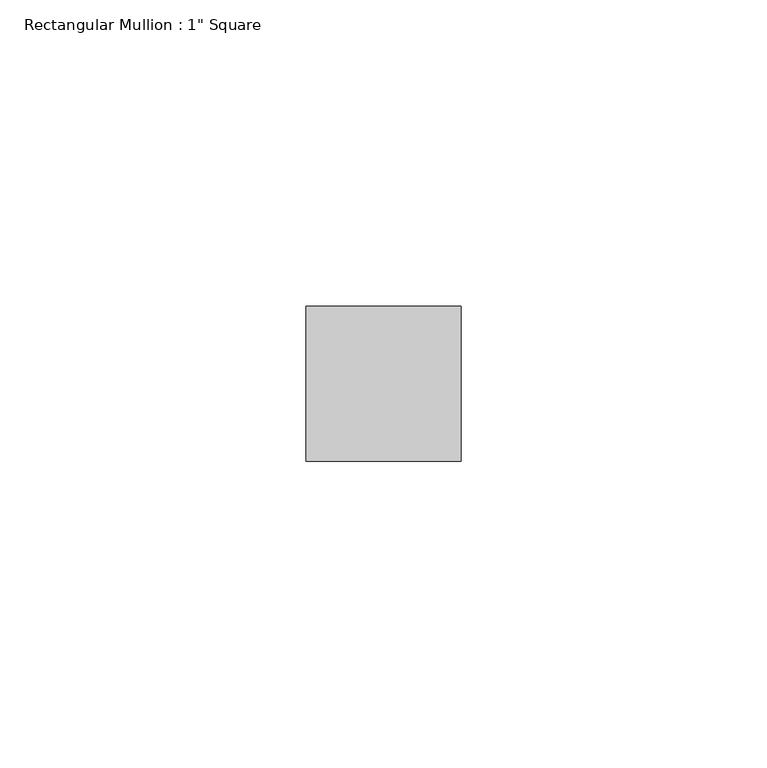
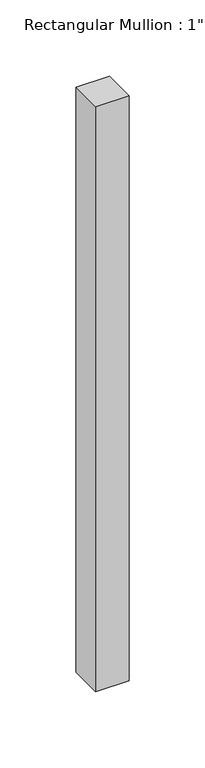
"""IFC4 building model written with IfcOpenShell, lengths in millimetres: member geometry."""

from ifc_helpers import new_model, si_unit, frame, origin, place, context, project, spatial, polyline, outline, extrude, source, transform, mapped, element, save


def member_0282b000(model_context):
    return source(origin(), model_context, "Body", "SweptSolid", [
        extrude(outline(polyline([(0.0, 12.7), (0.0, -12.7), (-25.4, -12.7), (-25.4, 12.7), (0.0, 12.7)])), frame((0.0, 0.0, -468.2712073), z_axis=(0.0, 0.0, 1.0), x_axis=(1.0, 0.0, 0.0)), (0.0, 0.0, 1.0), 468.2712073),
    ])


if __name__ == "__main__":
    model = new_model("IFC4")
    model_context = context("Model", 3, world=origin())
    ifc_project = project(units=[si_unit("LENGTHUNIT", "METRE", prefix="MILLI")], contexts=[model_context])
    site = spatial("IfcSite", under=ifc_project)
    building = spatial("IfcBuilding", under=site)
    placement = place(None, origin())
    member_shape = member_0282b000(model_context)
    element("IfcMember", 1, ObjectType="Rectangular Mullion : 1\" Square", at=placement, inside=building, context=model_context, shape_type="MappedRepresentation", body=[
        mapped(member_shape, transform((0.0, 0.0, 0.0), x_axis=(1.0, 0.0, 0.0), y_axis=(0.0, 1.0, 0.0), z_axis=(0.0, 0.0, 1.0))),
    ])
    save(model, "model.ifc")

# Revit data of these elements
# Type "Rectangular Mullion : 1\" Square"
#   built-in parameter 1007304 = 0.0833333 (stored number, unit not read)
#   built-in parameter 1007301 = 0.0416667 (stored number, unit not read)
#   built-in parameter 1007300 = 0.0416667 (stored number, unit not read)
# Element 1 (IfcMember, "Rectangular Mullion : 1\" Square")
#   Materials on its faces: "Metal - Aluminum"
# Materials
#   "Metal - Aluminum": class "Metal", colour RGB 247 247 247, transparency 0
